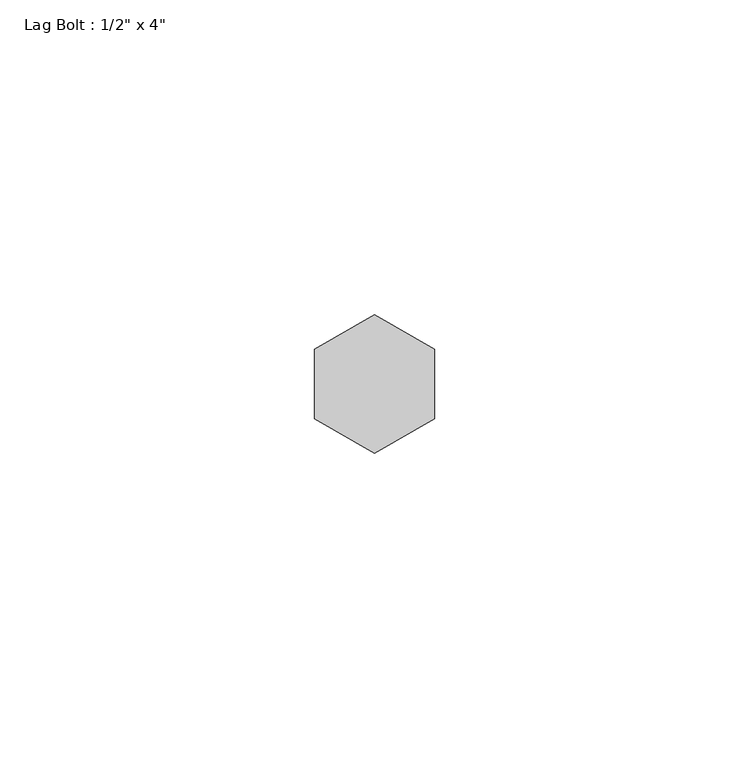
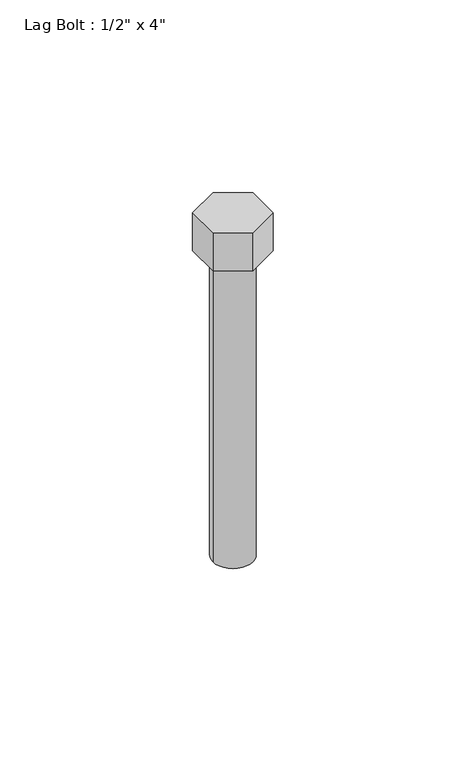
"""IFC4 building model written with IfcOpenShell, lengths in millimetres: proxy geometry."""

from ifc_helpers import new_model, si_unit, point, frame, origin, origin_with_axes, origin_2d, place, context, project, spatial, polyline, circle_curve, trimmed, segment, composite_curve, outline, extrude, source, transform, mapped, element, save


def proxy_b3a3e4df(model_context):
    return source(origin(), model_context, "Body", "SweptSolid", [
        extrude(outline(polyline([(-9.525, -5.4992613), (-9.525, 5.4992613), (0.0, 10.9985226), (9.525, 5.4992613), (9.525, -5.4992613), (0.0, -10.9985226), (-9.525, -5.4992613)])), origin_with_axes(), (0.0, 0.0, 1.0), 12.7),
        extrude(outline(composite_curve([segment(trimmed(circle_curve(origin_2d(), 6.35), [point((-6.35, 0.0))], [point((6.35, 0.0))], False, "CARTESIAN"), True, "CONTINUOUS"), segment(trimmed(circle_curve(origin_2d(), 6.35), [point((6.35, 0.0))], [point((-6.35, 0.0))], False, "CARTESIAN"), True, "CONTINUOUS")], self_intersect=False)), frame((0.0, 0.0, -101.6), z_axis=(0.0, 0.0, 1.0), x_axis=(1.0, 0.0, 0.0)), (0.0, 0.0, 1.0), 101.6),
    ])


if __name__ == "__main__":
    model = new_model("IFC4")
    model_context = context("Model", 3, world=origin())
    ifc_project = project(units=[si_unit("LENGTHUNIT", "METRE", prefix="MILLI")], contexts=[model_context])
    site = spatial("IfcSite", under=ifc_project)
    building = spatial("IfcBuilding", under=site)
    placement = place(None, origin())
    proxy_shape = proxy_b3a3e4df(model_context)
    element("IfcBuildingElementProxy", 1, Name="Lag Bolt : 1/2\" x 4\"", ObjectType="Lag Bolt : 1/2\" x 4\"", at=placement, inside=building, context=model_context, shape_type="MappedRepresentation", body=[
        mapped(proxy_shape, transform((0.0, 0.0, 0.0), x_axis=(1.0, 0.0, 0.0), y_axis=(0.0, 1.0, 0.0), z_axis=(0.0, 0.0, 1.0))),
    ])
    save(model, "model.ifc")

# Revit data of these elements
# Type "Lag Bolt : 1/2\" x 4\""
#   Thickness_of_Substrate [instance default] = 0' - 1"
#   Side = 0' - 0 111/256"
#   Radius = 0' - 0 1/4"
#   Length = 0' - 4"
#   Head Size = 0' - 0 3/4"
#   Head Radius = 0' - 0 3/8"
#   Head Height = 0' - 0 1/2"
#   Diameter = 0' - 0 1/2"
#   Default Elevation = 4' - 0"
#   Nut_Visibility [instance default] = no
#   Bolt Material (Size) [instance default] = none
